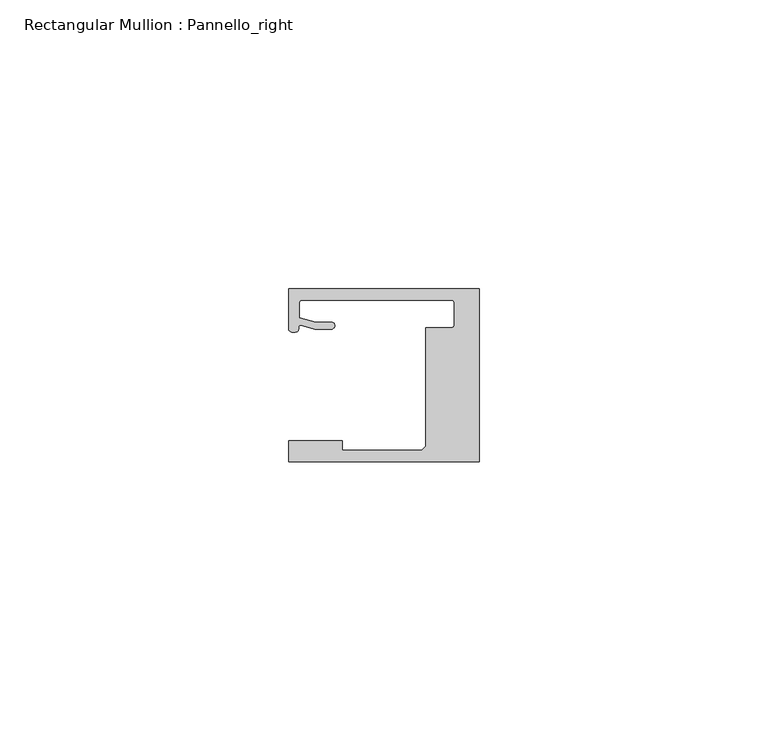
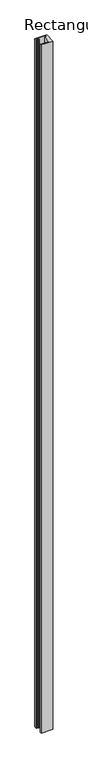
"""IFC4 building model written with IfcOpenShell, lengths in millimetres: member geometry, Rectangular Mullion : Pannello_right."""

from ifc_helpers import new_model, si_unit, frame, origin, place, context, project, spatial, polyline, circle_curve, source, transform, mapped, element, save
from ifc_brep_helpers import plane_surface, cylinder_surface, revolved_surface, extruded_surface, spline_curve, advanced_brep


def rectangular_mullion_pannello_right_492ebaf9(model_context):
    return source(origin(), model_context, "Body", "AdvancedBrep", [
        advanced_brep(
        [(-33.0, -15.0, 0.0), (0.0, -15.0, 0.0), (0.0, 15.0, 0.0), (-33.0000135, 15.0, 0.0), (-33.0000135, 8.0000472, 0.0), (-30.9223017, 8.6490241, 0.0), (-28.4999305, 7.9999523, 0.0), (-25.59998, 7.9999523, 0.0), (-25.59998, 9.1999523, 0.0), (-28.3419477, 9.1999523, 0.0), (-31.19998, 9.9657591, 0.0), (-31.19998, 12.50001, 0.0), (-30.69998, 13.00001, 0.0), (-4.7999726, 13.00001, 0.0), (-4.2999726, 12.50001, 0.0), (-4.2999726, 8.7500595, 0.0), (-4.7999726, 8.2500595, 0.0), (-9.2999726, 8.2500595, 0.0), (-9.2999726, -12.2999849, 0.0), (-10.0000103, -13.0000004, 0.0), (-23.700041, -13.0000004, 0.0), (-23.700041, -11.3000004, 0.0), (-33.0, -11.3000004, 0.0), (-33.0, -15.0, -2046.9999865), (-33.0, -11.3000004, -2046.9999865), (-23.700041, -11.3000004, -2046.9999865), (-23.700041, -13.0000004, -2046.9999865), (-10.0000103, -13.0000004, -2046.9999865), (-9.2999726, -12.2999849, -2046.9999865), (-9.2999726, 8.2500595, -2046.9999865), (-4.7999726, 8.2500595, -2046.9999865), (-4.2999726, 8.7500595, -2046.9999865), (-4.2999726, 12.50001, -2046.9999865), (-4.7999726, 13.00001, -2046.9999865), (-30.69998, 13.00001, -2046.9999865), (-31.19998, 12.50001, -2046.9999865), (-31.19998, 9.9657591, -2046.9999865), (-28.3419477, 9.1999523, -2046.9999865), (-25.59998, 9.1999523, -2046.9999865), (-25.59998, 7.9999523, -2046.9999865), (-28.4999305, 7.9999523, -2046.9999865), (-30.9223017, 8.6490241, -2046.9999865), (-33.0000135, 8.0000472, -2046.9999865), (-33.0000135, 15.0, -2046.9999865), (0.0, 15.0, -2046.9999865), (0.0, -15.0, -2046.9999865)],
        [
            (0, 1),
            (1, 2),
            (2, 3),
            (3, 4),
            (4, 5, spline_curve(3, [(-33.0000135, 8.0000472, 0.0), (-33.0000135, 7.457047519, 0.0), (-32.262327879, 7.456527435, 0.0), (-31.357433266, 7.563996614, 0.0), (-31.305645054, 7.690065204, 0.0), (-31.298563602, 8.366228555, 0.0), (-31.312054066, 8.717747958, 0.0), (-30.9223017, 8.6490241, 0.0)], [4, 2, 2, 4], [0.0, 0.0027053965905959043, 0.0058611956533709, 0.007702013405570312])),
            (5, 6),
            (6, 7),
            (7, 8, circle_curve(frame((-25.59998, 8.5999523, 0.0), z_axis=(0.0, 0.0, 1.0), x_axis=(0.0, 1.0, 0.0)), 0.6)),
            (8, 9),
            (9, 10),
            (10, 11),
            (11, 12, circle_curve(frame((-30.69998, 12.50001, 0.0), z_axis=(0.0, 0.0, -1.0), x_axis=(0.0, 1.0, 0.0)), 0.5)),
            (12, 13),
            (13, 14, circle_curve(frame((-4.7999726, 12.50001, 0.0), z_axis=(0.0, 0.0, -1.0), x_axis=(1.0, 0.0, 0.0)), 0.5)),
            (14, 15),
            (15, 16, circle_curve(frame((-4.7999726, 8.7500595, 0.0), z_axis=(0.0, 0.0, -1.0), x_axis=(0.0, -1.0, 0.0)), 0.5)),
            (16, 17),
            (17, 18),
            (18, 19),
            (19, 20),
            (20, 21),
            (21, 22),
            (22, 0),
            (23, 24),
            (24, 25),
            (25, 26),
            (26, 27),
            (27, 28),
            (28, 29),
            (29, 30),
            (30, 31, circle_curve(frame((-4.7999726, 8.7500595, -2046.9999865), z_axis=(0.0, 0.0, 1.0), x_axis=(0.0, -1.0, 0.0)), 0.5)),
            (31, 32),
            (32, 33, circle_curve(frame((-4.7999726, 12.50001, -2046.9999865), z_axis=(0.0, 0.0, 1.0), x_axis=(1.0, 0.0, 0.0)), 0.5)),
            (33, 34),
            (34, 35, circle_curve(frame((-30.69998, 12.50001, -2046.9999865), z_axis=(0.0, 0.0, 1.0), x_axis=(0.0, 1.0, 0.0)), 0.5)),
            (35, 36),
            (36, 37),
            (37, 38),
            (38, 39, circle_curve(frame((-25.59998, 8.5999523, -2046.9999865), z_axis=(0.0, 0.0, -1.0), x_axis=(0.0, 1.0, 0.0)), 0.6)),
            (39, 40),
            (40, 41),
            (41, 42, spline_curve(3, [(-30.9223017, 8.6490241, -2046.9999865), (-31.312054066, 8.717747958, -2046.9999865), (-31.298563602, 8.366228555, -2046.9999865), (-31.305645054, 7.690065204, -2046.9999865), (-31.357433266, 7.563996614, -2046.9999865), (-32.262327879, 7.456527435, -2046.9999865), (-33.0000135, 7.457047519, -2046.9999865), (-33.0000135, 8.0000472, -2046.9999865)], [4, 2, 2, 4], [0.0, 0.001840817752199412, 0.004996616814974408, 0.007702013405570312])),
            (42, 43),
            (43, 44),
            (44, 45),
            (45, 23),
            (0, 23),
            (45, 1),
            (44, 2),
            (43, 3),
            (42, 4),
            (41, 5),
            (40, 6),
            (39, 7),
            (38, 8),
            (37, 9),
            (36, 10),
            (35, 11),
            (34, 12),
            (33, 13),
            (32, 14),
            (31, 15),
            (30, 16),
            (29, 17),
            (28, 18),
            (27, 19),
            (26, 20),
            (25, 21),
            (24, 22),
        ],
        [
            plane_surface(frame((0.0, -36.2491502, 0.0), z_axis=(0.0, 0.0, 1.0), x_axis=(-1.0, 0.0, 0.0))),
            plane_surface(frame((0.0, -36.2491502, -2046.9999865), z_axis=(0.0, 0.0, -1.0), x_axis=(-1.0, 0.0, 0.0))),
            plane_surface(frame((-33.0, -15.0, 0.0), z_axis=(0.0, -1.0, 0.0), x_axis=(0.0, 0.0, -1.0))),
            plane_surface(frame((0.0, -15.0, 0.0), z_axis=(1.0, 0.0, 0.0), x_axis=(0.0, 0.0, -1.0))),
            plane_surface(frame((0.0, 15.0, 0.0), z_axis=(0.0, 1.0, 0.0), x_axis=(0.0, 0.0, -1.0))),
            plane_surface(frame((-33.0000135, 15.0, 0.0), z_axis=(-1.0, 0.0, 0.0), x_axis=(0.0, 0.0, -1.0))),
            extruded_surface(spline_curve(3, [(-33.0000135, 8.0000472, -2046.9999865), (-33.0000135, 7.457047519, -2046.9999865), (-32.262327879, 7.456527435, -2046.9999865), (-31.357433266, 7.563996614, -2046.9999865), (-31.305645054, 7.690065204, -2046.9999865), (-31.298563602, 8.366228555, -2046.9999865), (-31.312054066, 8.717747958, -2046.9999865), (-30.9223017, 8.6490241, -2046.9999865)], [4, 2, 2, 4], [0.0, 0.0027053965905959043, 0.0058611956533709, 0.007702013405570312]), (0.0, 0.0, 2046.9999865), 2046.9999865),
            plane_surface(frame((-30.9223017, 8.6490241, 0.0), z_axis=(-0.2588188320019168, -0.965925883389178, 0.0), x_axis=(0.0, 0.0, -1.0))),
            plane_surface(frame((-28.4999305, 7.9999523, 0.0), z_axis=(0.0, -1.0, 0.0), x_axis=(0.0, 0.0, -1.0))),
            cylinder_surface(frame((-25.59998, 8.5999523, 0.0), z_axis=(0.0, 0.0, 1.0), x_axis=(0.0, 1.0, 0.0)), 0.6),
            plane_surface(frame((-25.59998, 9.1999523, 0.0), z_axis=(0.0, 1.0, 0.0), x_axis=(0.0, 0.0, -1.0))),
            plane_surface(frame((-28.3419477, 9.1999523, 0.0), z_axis=(0.2588188320428738, 0.9659258833782035, 0.0), x_axis=(0.0, 0.0, -1.0))),
            plane_surface(frame((-31.19998, 9.9657591, 0.0), z_axis=(1.0, 0.0, 0.0), x_axis=(0.0, 0.0, -1.0))),
            revolved_surface(polyline([(-30.69998, 13.00001, -2046.9999865), (-30.69998, 13.00001, 0.0)]), (-30.69998, 12.50001, 0.0), (0.0, 0.0, -1.0)),
            plane_surface(frame((-30.69998, 13.00001, 0.0), z_axis=(0.0, -1.0, 0.0), x_axis=(0.0, 0.0, -1.0))),
            revolved_surface(polyline([(-4.2999726, 12.50001, -2046.9999865), (-4.2999726, 12.50001, 0.0)]), (-4.7999726, 12.50001, 0.0), (0.0, 0.0, -1.0)),
            plane_surface(frame((-4.2999726, 12.50001, 0.0), z_axis=(-1.0, 0.0, 0.0), x_axis=(0.0, 0.0, -1.0))),
            revolved_surface(polyline([(-4.7999726, 8.2500595, -2046.9999865), (-4.7999726, 8.2500595, 0.0)]), (-4.7999726, 8.7500595, 0.0), (0.0, 0.0, -1.0)),
            plane_surface(frame((-4.7999726, 8.2500595, 0.0), z_axis=(0.0, 1.0, 0.0), x_axis=(0.0, 0.0, -1.0))),
            plane_surface(frame((-9.2999726, 8.2500595, 0.0), z_axis=(-1.0, 0.0, 0.0), x_axis=(0.0, 0.0, -1.0))),
            plane_surface(frame((-9.2999726, -12.2999849, 0.0), z_axis=(-0.7070955486278075, 0.7071180135668587, 0.0), x_axis=(0.0, 0.0, -1.0))),
            plane_surface(frame((-10.0000103, -13.0000004, 0.0), z_axis=(0.0, 1.0, 0.0), x_axis=(0.0, 0.0, -1.0))),
            plane_surface(frame((-23.700041, -13.0000004, 0.0), z_axis=(1.0, 0.0, 0.0), x_axis=(0.0, 0.0, -1.0))),
            plane_surface(frame((-23.700041, -11.3000004, 0.0), z_axis=(0.0, 1.0, 0.0), x_axis=(0.0, 0.0, -1.0))),
            plane_surface(frame((-33.0, -11.3000004, 0.0), z_axis=(-1.0, 0.0, 0.0), x_axis=(0.0, 0.0, -1.0))),
        ],
        [
            (0, [[1, 2, 3, 4, 5, 6, 7, 8, 9, 10, 11, 12, 13, 14, 15, 16, 17, 18, 19, 20, 21, 22, 23]]),
            (1, [[24, 25, 26, 27, 28, 29, 30, 31, 32, 33, 34, 35, 36, 37, 38, 39, 40, 41, 42, 43, 44, 45, 46]]),
            (2, [[-1, 47, -46, 48]]),
            (3, [[-2, -48, -45, 49]]),
            (4, [[-3, -49, -44, 50]]),
            (5, [[-4, -50, -43, 51]]),
            (6, [[-5, -51, -42, 52]]),
            (7, [[-6, -52, -41, 53]]),
            (8, [[-7, -53, -40, 54]]),
            (9, [[-8, -54, -39, 55]]),
            (10, [[-9, -55, -38, 56]]),
            (11, [[-10, -56, -37, 57]]),
            (12, [[-11, -57, -36, 58]]),
            (13, [[-12, -58, -35, 59]]),
            (14, [[-13, -59, -34, 60]]),
            (15, [[-14, -60, -33, 61]]),
            (16, [[-15, -61, -32, 62]]),
            (17, [[-16, -62, -31, 63]]),
            (18, [[-17, -63, -30, 64]]),
            (19, [[-18, -64, -29, 65]]),
            (20, [[-19, -65, -28, 66]]),
            (21, [[-20, -66, -27, 67]]),
            (22, [[-21, -67, -26, 68]]),
            (23, [[-22, -68, -25, 69]]),
            (24, [[-23, -69, -24, -47]]),
        ],
    ),
    ])


if __name__ == "__main__":
    model = new_model("IFC4")
    model_context = context("Model", 3, world=origin())
    ifc_project = project(units=[si_unit("LENGTHUNIT", "METRE", prefix="MILLI")], contexts=[model_context])
    site = spatial("IfcSite", under=ifc_project)
    building = spatial("IfcBuilding", under=site)
    placement = place(None, origin())
    rectangular_mullion_pannello_right_shape = rectangular_mullion_pannello_right_492ebaf9(model_context)
    element("IfcMember", 1, ObjectType="Rectangular Mullion : Pannello_right", at=placement, inside=building, context=model_context, shape_type="MappedRepresentation", body=[
        mapped(rectangular_mullion_pannello_right_shape, transform((0.0, 0.0, 0.0), x_axis=(1.0, 0.0, 0.0), y_axis=(0.0, 1.0, 0.0), z_axis=(0.0, 0.0, 1.0))),
    ])
    save(model, "model.ifc")

# Revit data of these elements
# Type "Rectangular Mullion : Pannello_right"
#   built-in parameter 1007322 = 0.0984252 (stored number, unit not read)
#   built-in parameter 1007321 = 0.0305117 (stored number, unit not read)
#   built-in parameter 1007320 = 0 (stored number, unit not read)
